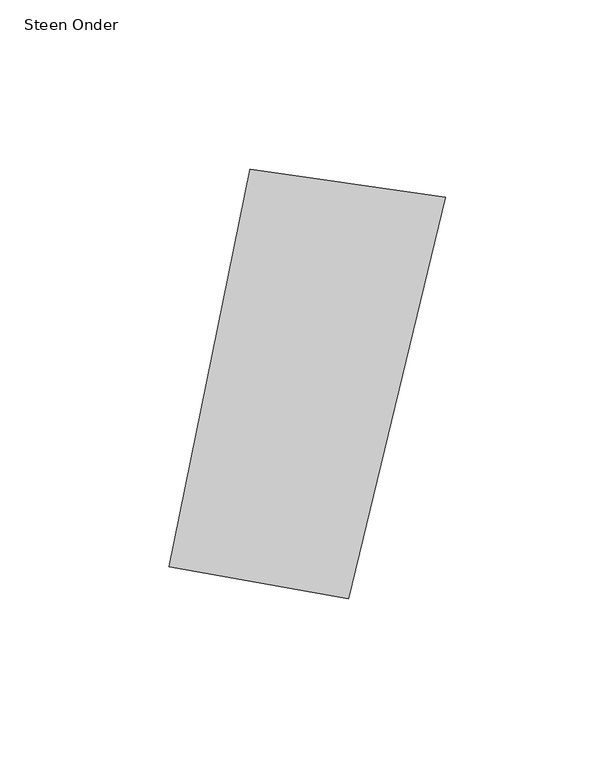
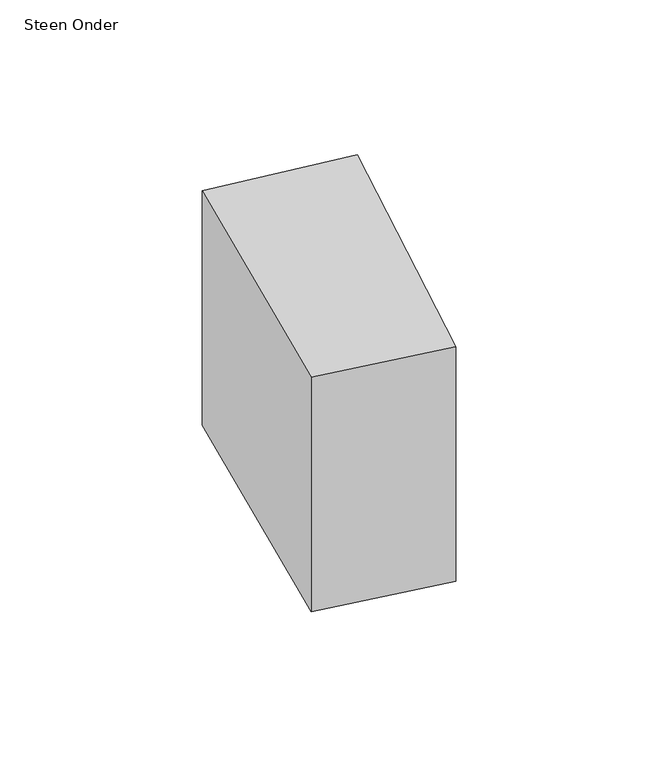
"""IFC4 building model written with IfcOpenShell, lengths in millimetres: proxy geometry, 00_GMA_steen_versie_4 : Steen Onder."""

from ifc_helpers import new_model, si_unit, origin, origin_with_axes, place, context, project, spatial, polyline, outline, extrude, source, transform, mapped, element, save


def steen_onder_1f40154c(model_context):
    return source(origin(), model_context, "Body", "SweptSolid", [
        extrude(outline(polyline([(114.3991338, 126.3169748), (85.7187697, 7.9279408), (32.7976741, 17.2471058), (56.5987729, 134.5606487), (114.3991338, 126.3169748)])), origin_with_axes(), (0.0, 0.0, 1.0), 100.0),
    ])


if __name__ == "__main__":
    model = new_model("IFC4")
    model_context = context("Model", 3, world=origin())
    ifc_project = project(units=[si_unit("LENGTHUNIT", "METRE", prefix="MILLI")], contexts=[model_context])
    site = spatial("IfcSite", under=ifc_project)
    building = spatial("IfcBuilding", under=site)
    placement = place(None, origin())
    steen_onder_shape = steen_onder_1f40154c(model_context)
    element("IfcBuildingElementProxy", 1, Name="00_GMA_steen_versie_4 : Steen Onder", ObjectType="00_GMA_steen_versie_4 : Steen Onder", at=placement, inside=building, context=model_context, shape_type="MappedRepresentation", body=[
        mapped(steen_onder_shape, transform((0.0, 0.0, 0.0), x_axis=(1.0, 0.0, 0.0), y_axis=(0.0, 1.0, 0.0), z_axis=(0.0, 0.0, 1.0))),
    ])
    save(model, "model.ifc")

# Revit data of these elements
# Type "00_GMA_steen_versie_4 : Steen Onder"
#   StootVoegHalfBoven [instance default] = 5 mm
#   StootVoegHalf [instance default] = 5 mm
#   StootVoegBreedteOnder = 10 mm
#   StootVoegBreedteBoven = 10 mm
#   Steendikte = 100 mm
#   LintVoegOnderHalf = 0 mm
#   LintVoegOnder = 0 mm
#   LintVoegBovenHalf = 5 mm
#   LintVoegBoven = 10 mm
#   materiaal = none
#   MateriaalVoeg = none
#   Default Elevation = 0
